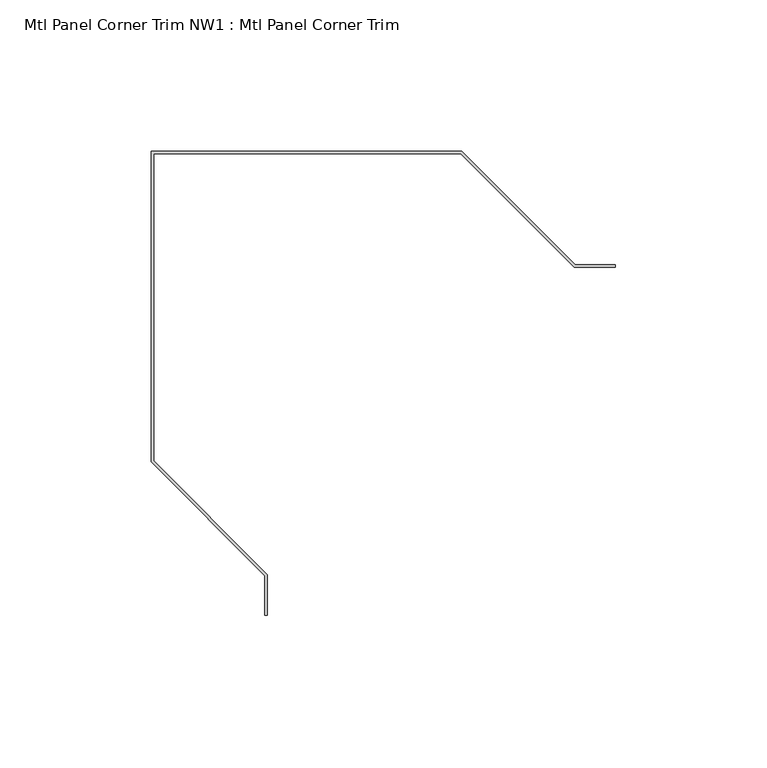
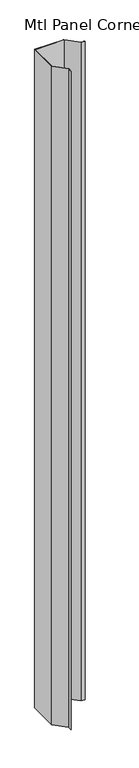
"""IFC4 building model written with IfcOpenShell, lengths in millimetres: proxy geometry, Mtl Panel Corner Trim NW1 : Mtl Panel Corner Trim."""

import ifcopenshell
import ifcopenshell.guid

model = None  # the IFC model being written
_history = None  # IfcOwnerHistory: only IFC2X3 demands one
_inside = {}  # id of a spatial element -> (the spatial element, [elements in it])
_under = {}  # id of a project, library or spatial element -> (it, [spatial elements below it])
_declared = {}  # id of a project -> (the project, [libraries it declares])
_typed = {}  # id of a type object -> (the type object, [elements of that type])
_made_of = {}  # id of a material, layer set ... -> (it, [elements and type objects made of it])


def new_model(schema):
    """Start an empty IFC model of exactly this schema.

    Asked for "IFC4X3", IfcOpenShell would pick the latest addendum, in which some entities
    have other attributes; the version numbers below select the first issue.
    IFC2X3 requires an IfcOwnerHistory on every rooted entity: one is made here for all.
    """
    global model, _history
    if schema == "IFC4X3":
        model = ifcopenshell.file(schema_version=(4, 3, 0, 0))
    else:
        model = ifcopenshell.file(schema=schema)
    _inside.clear()
    _under.clear()
    _declared.clear()
    _typed.clear()
    _made_of.clear()
    _history = None
    if model.schema == "IFC2X3":
        org = make("IfcOrganization", Name="unknown")
        user = make(
            "IfcPersonAndOrganization",
            ThePerson=make("IfcPerson", FamilyName="unknown"),
            TheOrganization=org,
        )
        app = make(
            "IfcApplication",
            ApplicationDeveloper=org,
            Version="unknown",
            ApplicationFullName="unknown",
            ApplicationIdentifier="unknown",
        )
        _history = make(
            "IfcOwnerHistory",
            OwningUser=user,
            OwningApplication=app,
            ChangeAction="ADDED",
            CreationDate=0,
        )
    return model


def make(cls, **values):
    """One entity of the class cls with the attributes given. An attribute that is None is left unset."""
    return model.create_entity(
        cls, **{name: value for name, value in values.items() if value is not None}
    )


def rooted(cls, **values):
    """An entity with a GlobalId (a new one), such as an element, a storey or a relation."""
    return make(cls, GlobalId=ifcopenshell.guid.new(), OwnerHistory=_history, **values)


def si_unit(unit_type, name, prefix=None):
    """IfcSIUnit, for example si_unit("LENGTHUNIT", "METRE", prefix="MILLI")."""
    return make("IfcSIUnit", UnitType=unit_type, Prefix=prefix, Name=name)


def assignment(units):
    """IfcUnitAssignment: the units of a project."""
    return None if units is None else make("IfcUnitAssignment", Units=units)


def point(xyz):
    """IfcCartesianPoint."""
    return None if xyz is None else make("IfcCartesianPoint", Coordinates=xyz)


def direction(xyz):
    """IfcDirection."""
    return None if xyz is None else make("IfcDirection", DirectionRatios=xyz)


def frame(location, z_axis=None, x_axis=None):
    """IfcAxis2Placement3D, a coordinate frame: its origin and axes. An axis left out is left unset."""
    return make(
        "IfcAxis2Placement3D",
        Location=point(location),
        Axis=direction(z_axis),
        RefDirection=direction(x_axis),
    )


def origin():
    """The frame at (0, 0, 0) with its axes left unset."""
    return frame((0.0, 0.0, 0.0))


def place(relative_to, where):
    """IfcLocalPlacement: puts the frame where relative to a parent placement (None: the world)."""
    return make(
        "IfcLocalPlacement", PlacementRelTo=relative_to, RelativePlacement=where
    )


def context(
    kind, dimensions, precision=None, world=None, true_north=None, identifier=None
):
    """IfcGeometricRepresentationContext, for example the 3D "Model" context."""
    return make(
        "IfcGeometricRepresentationContext",
        ContextIdentifier=identifier,
        ContextType=kind,
        CoordinateSpaceDimension=dimensions,
        Precision=precision,
        WorldCoordinateSystem=world,
        TrueNorth=true_north,
    )


def project(units=None, contexts=None):
    """IfcProject with its units and contexts."""
    return rooted(
        "IfcProject",
        Name="project",
        RepresentationContexts=contexts,
        UnitsInContext=assignment(units),
    )


def spatial(cls, under=None, at=None, **own):
    """A site, building, storey or space (cls), placed at a placement, below another one or the project."""
    s = rooted(cls, ObjectPlacement=at, **own)
    if under is not None:
        _under.setdefault(under.id(), (under, []))[1].append(s)
    return s


def polyline(points):
    """IfcPolyline through the points."""
    return make("IfcPolyline", Points=[point(p) for p in points])


def outline(outer, holes=None, kind="AREA"):
    """IfcArbitraryClosedProfileDef: a profile drawn as a closed curve; with holes, ...WithVoids."""
    if holes is None:
        return make("IfcArbitraryClosedProfileDef", ProfileType=kind, OuterCurve=outer)
    return make(
        "IfcArbitraryProfileDefWithVoids",
        ProfileType=kind,
        OuterCurve=outer,
        InnerCurves=holes,
    )


def extrude(swept, where, along, depth):
    """IfcExtrudedAreaSolid: the profile swept, set in the frame where, extruded along a direction by depth."""
    return make(
        "IfcExtrudedAreaSolid",
        SweptArea=swept,
        Position=where,
        ExtrudedDirection=direction(along),
        Depth=depth,
    )


def shape(context_of_items, identifier, shape_type, items):
    """IfcShapeRepresentation: the items that make up one representation, for example the "Body"."""
    return make(
        "IfcShapeRepresentation",
        ContextOfItems=context_of_items,
        RepresentationIdentifier=identifier,
        RepresentationType=shape_type,
        Items=items,
    )


def source(mapping_origin, context_of_items, identifier, shape_type, items):
    """IfcRepresentationMap: a shape defined once, which mapped items show again and again."""
    return make(
        "IfcRepresentationMap",
        MappingOrigin=mapping_origin,
        MappedRepresentation=shape(context_of_items, identifier, shape_type, items),
    )


def transform(
    local_origin,
    x_axis=None,
    y_axis=None,
    z_axis=None,
    scale=None,
    scale2=None,
    scale3=None,
    uniform=True,
):
    """IfcCartesianTransformationOperator3D, or its non-uniform kind. x_axis, y_axis, z_axis: its Axis1, 2, 3."""
    if uniform:
        return make(
            "IfcCartesianTransformationOperator3D",
            Axis1=direction(x_axis),
            Axis2=direction(y_axis),
            LocalOrigin=point(local_origin),
            Scale=scale,
            Axis3=direction(z_axis),
        )
    return make(
        "IfcCartesianTransformationOperator3DnonUniform",
        Axis1=direction(x_axis),
        Axis2=direction(y_axis),
        LocalOrigin=point(local_origin),
        Scale=scale,
        Axis3=direction(z_axis),
        Scale2=scale2,
        Scale3=scale3,
    )


def mapped(mapping_source, mapping_target):
    """IfcMappedItem: shows the shape of a source again, moved by a transform."""
    return make(
        "IfcMappedItem", MappingSource=mapping_source, MappingTarget=mapping_target
    )


def made_of(thing, what):
    """Note that an element or type object is made of a material, layer set ...; save() writes the relation."""
    if what is not None:
        _made_of.setdefault(what.id(), (what, []))[1].append(thing)
    return thing


def element(
    cls,
    number,
    at=None,
    inside=None,
    cuts=None,
    type_object=None,
    material=None,
    context=None,
    identifier="Body",
    shape_type=None,
    held_by="IfcProductDefinitionShape",
    body=None,
    shapes=None,
    **own,
):
    """One element of the class cls, such as IfcWall. Its Tag is "e" and its number.

    at: its placement. inside: the storey or other place that contains it. cuts: it is an
    opening in that element (IfcRelVoidsElement). A single representation is given by context,
    identifier, shape_type and body (its items); several are given by shapes. held_by: the class
    of the entity that holds the representations. save() writes the other relations.
    """
    e = rooted(cls, Tag="e%d" % number, ObjectPlacement=at, **own)
    if body is not None:
        shapes = [shape(context, identifier, shape_type, body)]
    if shapes is not None:
        e.Representation = make(held_by, Representations=shapes)
    if inside is not None:
        _inside.setdefault(inside.id(), (inside, []))[1].append(e)
    if cuts is not None:
        rooted(
            "IfcRelVoidsElement", RelatingBuildingElement=cuts, RelatedOpeningElement=e
        )
    if type_object is not None:
        _typed.setdefault(type_object.id(), (type_object, []))[1].append(e)
    return made_of(e, material)


def aggregate(whole, parts):
    """IfcRelAggregates: a whole, such as a stair, and the parts it consists of."""
    return rooted("IfcRelAggregates", RelatingObject=whole, RelatedObjects=parts)


def save(model, path):
    """Write the relations noted so far, then the file.

    IfcRelAggregates (storeys below a building ...), IfcRelContainedInSpatialStructure (elements
    in a storey), IfcRelDefinesByType, IfcRelAssociatesMaterial and IfcRelDeclares: one each for
    every whole, place, type object, material and project.
    """
    for whole, parts in _under.values():
        aggregate(whole, parts)
    for where, things in _inside.values():
        rooted(
            "IfcRelContainedInSpatialStructure",
            RelatedElements=things,
            RelatingStructure=where,
        )
    for kind, things in _typed.values():
        rooted("IfcRelDefinesByType", RelatedObjects=things, RelatingType=kind)
    for what, things in _made_of.values():
        rooted("IfcRelAssociatesMaterial", RelatedObjects=things, RelatingMaterial=what)
    for by, libraries in _declared.values():
        rooted("IfcRelDeclares", RelatingContext=by, RelatedDefinitions=libraries)
    model.write(path)


def mtl_panel_corner_trim_nw1_mtl_panel_corner_trim_15613486(model_context):
    return source(origin(), model_context, "Body", "SweptSolid", [
        extrude(outline(polyline([(587365.3854739, -531753.7703841), (587364.5980739, -531753.7703841), (587364.5980739, -531740.6345358), (587327.0060739, -531703.0425358), (587327.0060739, -531600.3289841), (587429.7196257, -531600.3289841), (587467.2100257, -531637.8193841), (587480.4474739, -531637.8193841), (587480.4474739, -531638.6131341), (587466.8812437, -531638.6131341), (587429.3908437, -531601.1227341), (587327.7998239, -531601.1227341), (587327.7998239, -531702.7137538), (587365.3854739, -531740.2994038), (587365.3854739, -531753.7703841)])), frame((0.0, 0.0, 6.35), z_axis=(0.0, 0.0, 1.0), x_axis=(1.0, 0.0, 0.0)), (0.0, 0.0, 1.0), 2432.05),
    ])


if __name__ == "__main__":
    model = new_model("IFC4")
    model_context = context("Model", 3, world=origin())
    ifc_project = project(units=[si_unit("LENGTHUNIT", "METRE", prefix="MILLI")], contexts=[model_context])
    site = spatial("IfcSite", under=ifc_project)
    building = spatial("IfcBuilding", under=site)
    placement = place(None, origin())
    mtl_panel_corner_trim_nw1_mtl_panel_corner_trim_shape = mtl_panel_corner_trim_nw1_mtl_panel_corner_trim_15613486(model_context)
    element("IfcBuildingElementProxy", 1, Name="Mtl Panel Corner Trim NW1 : Mtl Panel Corner Trim", ObjectType="Mtl Panel Corner Trim NW1 : Mtl Panel Corner Trim", at=placement, inside=building, context=model_context, shape_type="MappedRepresentation", body=[
        mapped(mtl_panel_corner_trim_nw1_mtl_panel_corner_trim_shape, transform((0.0, 0.0, 0.0), x_axis=(1.0, 0.0, 0.0), y_axis=(0.0, 1.0, 0.0), z_axis=(0.0, 0.0, 1.0))),
    ])
    save(model, "model.ifc")

# Revit data of these elements
# Element 1 (IfcBuildingElementProxy, "Mtl Panel Corner Trim NW1 : Mtl Panel Corner Trim")
#   Materials on its faces: "CORNER TRIM BY MTL PANEL MFR."
# Materials
#   "CORNER TRIM BY MTL PANEL MFR.": class "Generic", colour RGB 239 242 240, transparency 0, Cost = 0
